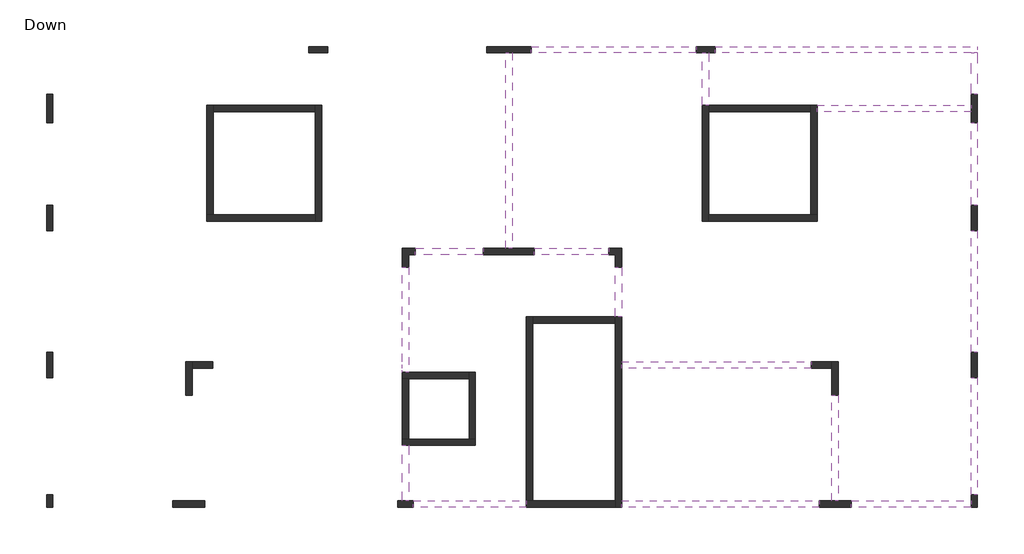
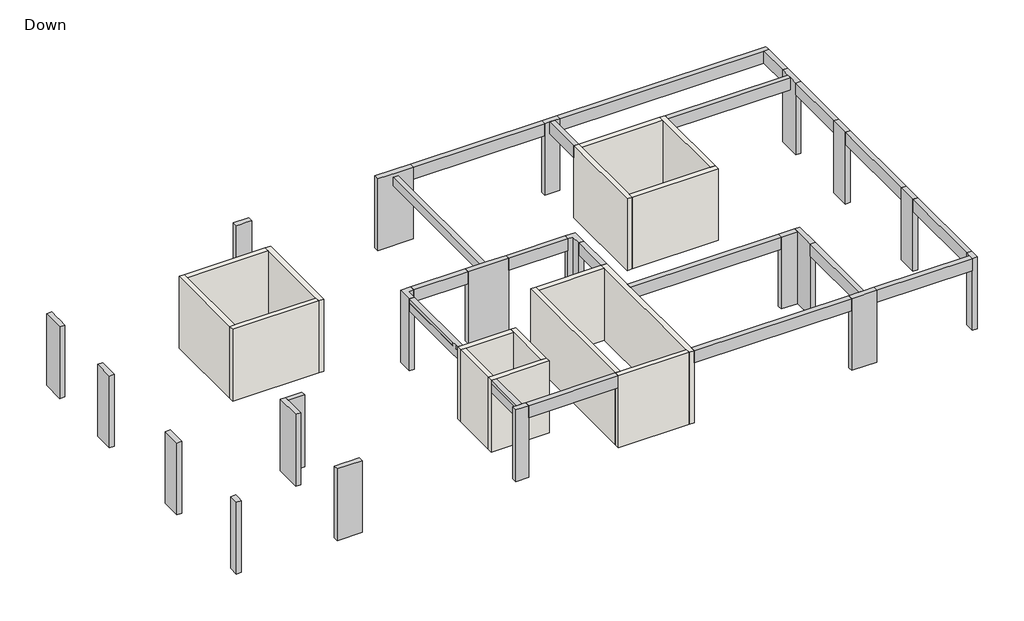
# One storey: 21 columns, 19 beams, 16 walls.
# Revit data of these elements (continued)
# Element 39 (IfcColumn, "L Column : 20/40/20/20")
#   Comments = ""
#   Mark = "C20"
#   SOFiSTiK_AMG_Comments = ""
#   SOFiSTiK_AMG_Scheduled = yes
#   SOFiSTiK_AMG_Adjusted = yes
#   Structural Material = Concrete
#   Phase Created = New Construction
# Element 40 (IfcColumn, "L Column : 20/40/20/20")
#   Comments = ""
#   Mark = "C21"
#   SOFiSTiK_AMG_Comments = ""
#   SOFiSTiK_AMG_Scheduled = yes
#   SOFiSTiK_AMG_Adjusted = yes
#   Structural Material = Concrete
#   Phase Created = New Construction
# Element 41 (IfcWall, "20")
#   Comments = ""
#   Mark = "W1"
#   SOFiSTiK_EdgeZones = "W1"
#   SOFiSTiK_AMG_Comments = ""
#   Top Offset = 0 cm
#   Base Offset = 0 cm
#   wall height = 300 cm
#   SOFiSTiK_AMG_Scheduled = yes
#   SOFiSTiK_AMG_Adjusted = yes
#   Phase Created = New Construction
#   Base Constraint = Down
#   Top Constraint = Typical Floor
#   Materials on its faces: "Concrete"
# Element 42 (IfcWall, "20")
#   Comments = ""
#   Mark = "W2"
#   SOFiSTiK_EdgeZones = "W2"
#   SOFiSTiK_AMG_Comments = ""
#   Top Offset = 0 cm
#   Base Offset = 0 cm
#   wall height = 300 cm
#   SOFiSTiK_AMG_Scheduled = yes
#   SOFiSTiK_AMG_Adjusted = yes
#   Phase Created = New Construction
#   Base Constraint = Down
#   Top Constraint = Typical Floor
#   Materials on its faces: "Concrete"
# Element 43 (IfcWall, "20")
#   Comments = ""
#   Mark = "W3"
#   SOFiSTiK_EdgeZones = "W3"
#   SOFiSTiK_AMG_Comments = ""
#   Top Offset = 0 cm
#   Base Offset = 0 cm
#   wall height = 300 cm
#   SOFiSTiK_AMG_Scheduled = yes
#   SOFiSTiK_AMG_Adjusted = yes
#   Phase Created = New Construction
#   Base Constraint = Down
#   Top Constraint = Typical Floor
#   Materials on its faces: "Concrete"
# Element 44 (IfcWall, "20")
#   Comments = ""
#   Mark = "W4"
#   SOFiSTiK_EdgeZones = "W4"
#   SOFiSTiK_AMG_Comments = ""
#   Top Offset = 0 cm
#   Base Offset = 0 cm
#   wall height = 300 cm
#   SOFiSTiK_AMG_Scheduled = yes
#   SOFiSTiK_AMG_Adjusted = yes
#   Phase Created = New Construction
#   Base Constraint = Down
#   Top Constraint = Typical Floor
#   Materials on its faces: "Concrete"
# Element 45 (IfcWall, "20")
#   Comments = ""
#   Mark = "W5"
#   SOFiSTiK_EdgeZones = "W5"
#   SOFiSTiK_AMG_Comments = ""
#   Top Offset = 0 cm
#   Base Offset = 0 cm
#   wall height = 300 cm
#   SOFiSTiK_AMG_Scheduled = yes
#   SOFiSTiK_AMG_Adjusted = yes
#   Phase Created = New Construction
#   Base Constraint = Down
#   Top Constraint = Typical Floor
#   Materials on its faces: "Concrete"
# Element 46 (IfcWall, "20")
#   Comments = ""
#   Mark = "W6"
#   SOFiSTiK_EdgeZones = "W6"
#   SOFiSTiK_AMG_Comments = ""
#   Top Offset = 0 cm
#   Base Offset = 0 cm
#   wall height = 300 cm
#   SOFiSTiK_AMG_Scheduled = yes
#   SOFiSTiK_AMG_Adjusted = yes
#   Phase Created = New Construction
#   Base Constraint = Down
#   Top Constraint = Typical Floor
#   Materials on its faces: "Concrete"
# Element 47 (IfcWall, "20")
#   Comments = ""
#   Mark = "W7"
#   SOFiSTiK_EdgeZones = "W7"
#   SOFiSTiK_AMG_Comments = ""
#   Top Offset = 0 cm
#   Base Offset = 0 cm
#   wall height = 300 cm
#   SOFiSTiK_AMG_Scheduled = yes
#   SOFiSTiK_AMG_Adjusted = yes
#   Phase Created = New Construction
#   Base Constraint = Down
#   Top Constraint = Typical Floor
#   Materials on its faces: "Concrete"
# Element 48 (IfcWall, "20")
#   Comments = ""
#   Mark = "W8"
#   SOFiSTiK_EdgeZones = "W8"
#   SOFiSTiK_AMG_Comments = ""
#   Top Offset = 0 cm
#   Base Offset = 0 cm
#   wall height = 300 cm
#   SOFiSTiK_AMG_Scheduled = yes
#   SOFiSTiK_AMG_Adjusted = yes
#   Phase Created = New Construction
#   Base Constraint = Down
#   Top Constraint = Typical Floor
#   Materials on its faces: "Concrete"
# Element 49 (IfcWall, "20")
#   Comments = ""
#   Mark = "W9"
#   SOFiSTiK_EdgeZones = "W9"
#   SOFiSTiK_AMG_Comments = ""
#   Top Offset = 0 cm
#   Base Offset = 0 cm
#   wall height = 300 cm
#   SOFiSTiK_AMG_Scheduled = yes
#   SOFiSTiK_AMG_Adjusted = yes
#   Phase Created = New Construction
#   Base Constraint = Down
#   Top Constraint = Typical Floor
#   Materials on its faces: "Concrete"
# Element 50 (IfcWall, "20")
#   Comments = ""
#   Mark = "W10"
#   SOFiSTiK_EdgeZones = "W10"
#   SOFiSTiK_AMG_Comments = ""
#   Top Offset = 0 cm
#   Base Offset = 0 cm
#   wall height = 300 cm
#   SOFiSTiK_AMG_Scheduled = yes
#   SOFiSTiK_AMG_Adjusted = yes
#   Phase Created = New Construction
#   Base Constraint = Down
#   Top Constraint = Typical Floor
#   Materials on its faces: "Concrete"
# Element 51 (IfcWall, "20")
#   Comments = ""
#   Mark = "W11"
#   SOFiSTiK_EdgeZones = "W11"
#   SOFiSTiK_AMG_Comments = ""
#   Top Offset = 0 cm
#   Base Offset = 0 cm
#   wall height = 300 cm
#   SOFiSTiK_AMG_Scheduled = yes
#   SOFiSTiK_AMG_Adjusted = yes
#   Phase Created = New Construction
#   Base Constraint = Down
#   Top Constraint = Typical Floor
#   Materials on its faces: "Concrete"
# Element 52 (IfcWall, "20")
#   Comments = ""
#   Mark = "W12"
#   SOFiSTiK_EdgeZones = "W12"
#   SOFiSTiK_AMG_Comments = ""
#   Top Offset = 0 cm
#   Base Offset = 0 cm
#   wall height = 300 cm
#   SOFiSTiK_AMG_Scheduled = yes
#   SOFiSTiK_AMG_Adjusted = yes
#   Phase Created = New Construction
#   Base Constraint = Down
#   Top Constraint = Typical Floor
#   Materials on its faces: "Concrete"
# Element 53 (IfcWall, "20")
#   Comments = ""
#   Mark = "W13"
#   SOFiSTiK_EdgeZones = "W13"
#   SOFiSTiK_AMG_Comments = ""
#   Top Offset = 0 cm
#   Base Offset = 0 cm
#   wall height = 300 cm
#   SOFiSTiK_AMG_Scheduled = yes
#   SOFiSTiK_AMG_Adjusted = yes
#   Phase Created = New Construction
#   Base Constraint = Down
#   Top Constraint = Typical Floor
#   Materials on its faces: "Concrete"
# Element 54 (IfcWall, "20")
#   Comments = ""
#   Mark = "W14"
#   SOFiSTiK_EdgeZones = "W14"
#   SOFiSTiK_AMG_Comments = ""
#   Top Offset = 0 cm
#   Base Offset = 0 cm
#   wall height = 300 cm
#   SOFiSTiK_AMG_Scheduled = yes
#   SOFiSTiK_AMG_Adjusted = yes
#   Phase Created = New Construction
#   Base Constraint = Down
#   Top Constraint = Typical Floor
#   Materials on its faces: "Concrete"
# Element 55 (IfcWall, "20")
#   Comments = ""
#   Mark = "W15"
#   SOFiSTiK_EdgeZones = "W15"
#   SOFiSTiK_AMG_Comments = ""
#   Top Offset = 0 cm
#   Base Offset = 0 cm
#   wall height = 300 cm
#   SOFiSTiK_AMG_Scheduled = yes
#   SOFiSTiK_AMG_Adjusted = yes
#   Phase Created = New Construction
#   Base Constraint = Down
#   Top Constraint = Typical Floor
#   Materials on its faces: "Concrete"
# Element 56 (IfcWall, "20")
#   Comments = ""
#   Mark = "W16"
#   SOFiSTiK_EdgeZones = "W16"
#   SOFiSTiK_AMG_Comments = ""
#   Top Offset = 0 cm
#   Base Offset = 0 cm
#   wall height = 300 cm
#   SOFiSTiK_AMG_Scheduled = yes
#   SOFiSTiK_AMG_Adjusted = yes
#   Phase Created = New Construction
#   Base Constraint = Down
#   Top Constraint = Typical Floor
#   Materials on its faces: "Concrete"
# Materials
#   "Concrete": class "Concrete", colour RGB 192 192 192, transparency 0, Keynote = "01000", Description = "Cast-in-place concrete", Cost = 0
#   "Concrete, Cast-in-Place gray": class "Concrete", colour RGB 192 192 192, transparency 0, Description = "Cast-in-place concrete", Cost = 0
